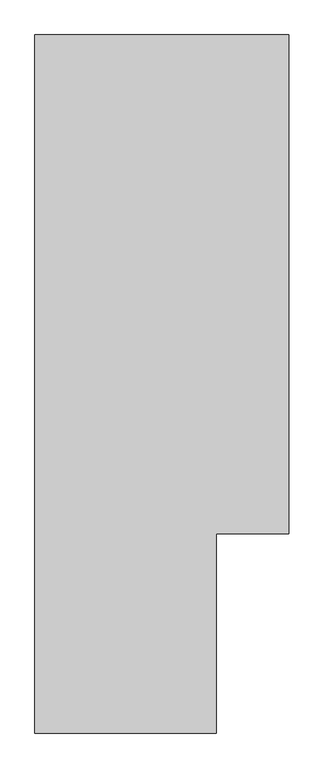
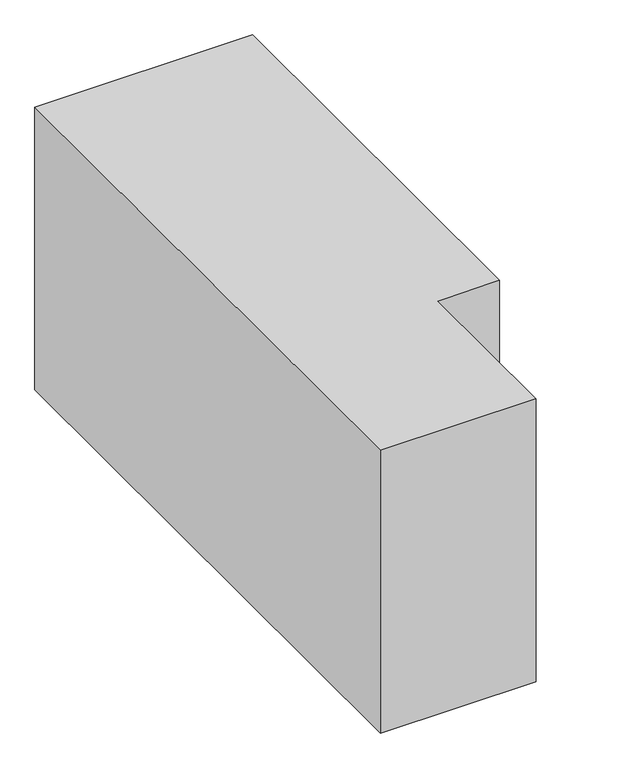
"""IFC4 building model written with IfcOpenShell, lengths in millimetres: proxy geometry, 0_3d_modell."""

from ifc_helpers import new_model, si_unit, origin, origin_with_axes, place, context, project, spatial, polyline, outline, extrude, source, transform, mapped, element, save


def generic_models_18af1c3a(model_context):
    return source(origin(), model_context, "Body", "SweptSolid", [
        extrude(outline(polyline([(2100.0, 5772.0), (2100.0, 1646.0204176), (1500.0, 1646.0204176), (1500.0, 0.0), (0.0, 0.0), (0.0, 5772.0), (2100.0, 5772.0)])), origin_with_axes(), (0.0, 0.0, 1.0), 2880.0),
    ])


if __name__ == "__main__":
    model = new_model("IFC4")
    model_context = context("Model", 3, world=origin())
    ifc_project = project(units=[si_unit("LENGTHUNIT", "METRE", prefix="MILLI")], contexts=[model_context])
    site = spatial("IfcSite", under=ifc_project)
    building = spatial("IfcBuilding", under=site)
    placement = place(None, origin())
    generic_models_shape = generic_models_18af1c3a(model_context)
    element("IfcBuildingElementProxy", 1, Name="0_3d_modell", ObjectType="0_3d_modell", at=placement, inside=building, context=model_context, shape_type="MappedRepresentation", body=[
        mapped(generic_models_shape, transform((0.0, 0.0, 0.0), x_axis=(1.0, 0.0, 0.0), y_axis=(0.0, 1.0, 0.0), z_axis=(0.0, 0.0, 1.0))),
    ])
    save(model, "model.ifc")

# Revit data of these elements
# Element 1 (IfcBuildingElementProxy, "0_3d_modell")
#   Materials on its faces: "*1"
# Materials
#   "*1": class "Unassigned", colour RGB 175 175 175, transparency 0
